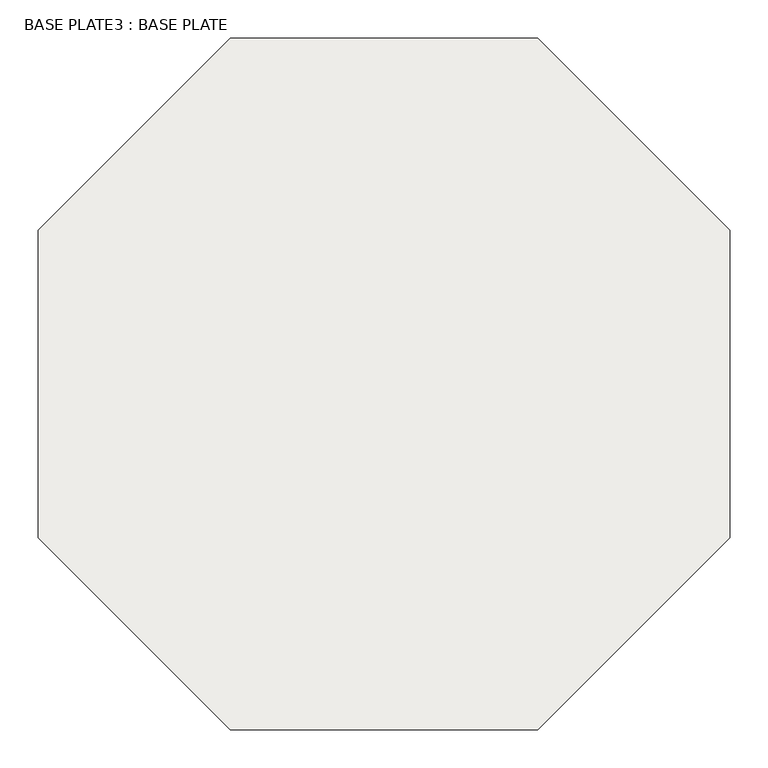
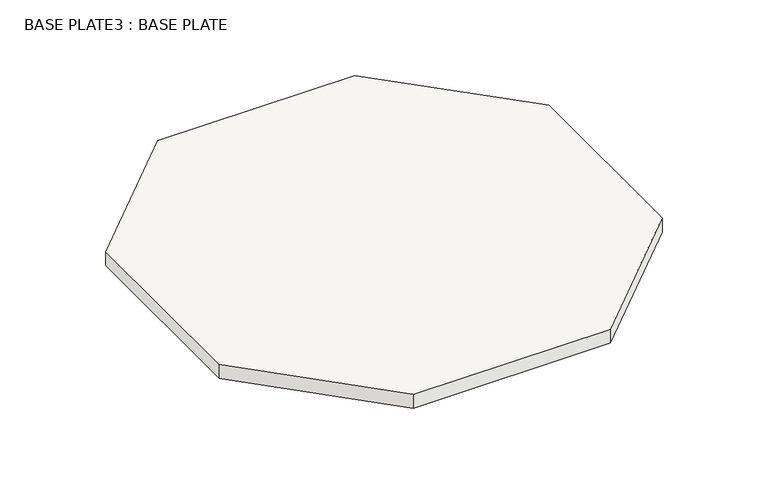
"""IFC4 building model written with IfcOpenShell, lengths in millimetres: slab geometry, BASE PLATE3 : BASE PLATE."""

from ifc_helpers import new_model, si_unit, frame, origin, place, context, project, spatial, polyline, outline, extrude, source, transform, mapped, element, save


def base_plate3_base_plate_0440a609(model_context):
    return source(origin(), model_context, "Body", "SweptSolid", [
        extrude(outline(polyline([(-495.7763606, -7383.9705533), (-495.7763606, -7783.9705533), (-745.7763606, -8033.9705533), (-1145.7763606, -8033.9705533), (-1395.7763606, -7783.9705533), (-1395.7763606, -7383.9705533), (-1145.7763606, -7133.9705533), (-745.7763606, -7133.9705533), (-495.7763606, -7383.9705533)])), frame((0.0, 0.0, 160.0), z_axis=(0.0, 0.0, 1.0), x_axis=(1.0, 0.0, 0.0)), (0.0, 0.0, 1.0), 30.0),
    ])


if __name__ == "__main__":
    model = new_model("IFC4")
    model_context = context("Model", 3, world=origin())
    ifc_project = project(units=[si_unit("LENGTHUNIT", "METRE", prefix="MILLI")], contexts=[model_context])
    site = spatial("IfcSite", under=ifc_project)
    building = spatial("IfcBuilding", under=site)
    placement = place(None, origin())
    base_plate3_base_plate_shape = base_plate3_base_plate_0440a609(model_context)
    element("IfcSlab", 1, ObjectType="BASE PLATE3 : BASE PLATE", at=placement, inside=building, context=model_context, shape_type="MappedRepresentation", body=[
        mapped(base_plate3_base_plate_shape, transform((0.0, 0.0, 0.0), x_axis=(1.0, 0.0, 0.0), y_axis=(0.0, 1.0, 0.0), z_axis=(0.0, 0.0, 1.0))),
    ])
    save(model, "model.ifc")
